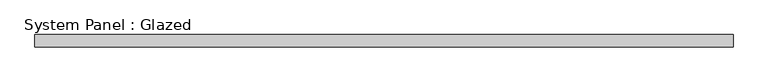
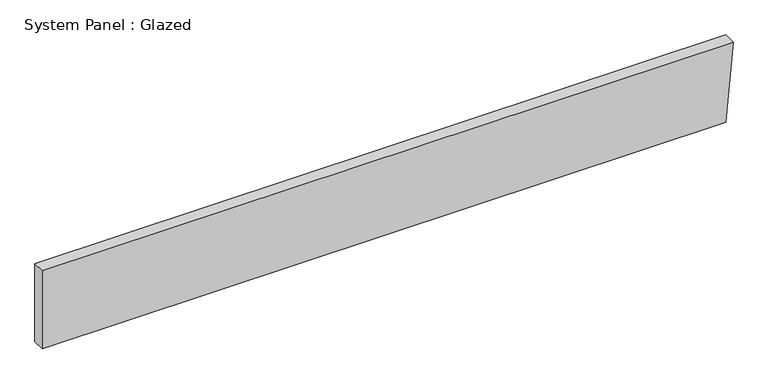
"""IFC4 building model written with IfcOpenShell, lengths in millimetres: plate geometry, System Panel : Glazed."""

from ifc_helpers import new_model, si_unit, frame, origin, place, context, project, spatial, polyline, outline, extrude, source, transform, mapped, element, save


def system_panel_glazed_9c30f1a4(model_context):
    return source(origin(), model_context, "Body", "SweptSolid", [
        extrude(outline(polyline([(0.0, -708.5978036), (0.0, 694.0133132), (169.2731269, 708.5978036), (169.2731269, -708.5978036), (0.0, -708.5978036)])), frame((0.0, -44.45, 0.0), z_axis=(0.0, 1.0, 0.0), x_axis=(0.0, 0.0, 1.0)), (0.0, 0.0, 1.0), 25.4),
    ])


if __name__ == "__main__":
    model = new_model("IFC4")
    model_context = context("Model", 3, world=origin())
    ifc_project = project(units=[si_unit("LENGTHUNIT", "METRE", prefix="MILLI")], contexts=[model_context])
    site = spatial("IfcSite", under=ifc_project)
    building = spatial("IfcBuilding", under=site)
    placement = place(None, origin())
    system_panel_glazed_shape = system_panel_glazed_9c30f1a4(model_context)
    element("IfcPlate", 1, ObjectType="System Panel : Glazed", at=placement, inside=building, context=model_context, shape_type="MappedRepresentation", body=[
        mapped(system_panel_glazed_shape, transform((0.0, 0.0, 0.0), x_axis=(1.0, 0.0, 0.0), y_axis=(0.0, 1.0, 0.0), z_axis=(0.0, 0.0, 1.0))),
    ])
    save(model, "model.ifc")

# Revit data of these elements
# Type "System Panel : Glazed"
#   Construction Type Id = "GSP4R"
#   Analytic Construction = "1/8 in Pilkington single glazing"
#   Visual Light Transmittance = 0.9
#   Solar Heat Gain Coefficient = 0.86
#   Heat Transfer Coefficient (U) = 1.18115 BTU/(h·ft²·°F)
#   Define Thermal Properties by = 1
# Element 1 (IfcPlate, "System Panel : Glazed")
#   Materials on its faces: "Glass"
# Materials
#   "Glass": class "Glass", colour RGB 0 128 192, transparency 0.75, Description = "Soda Lime Glass", Cost = 0
